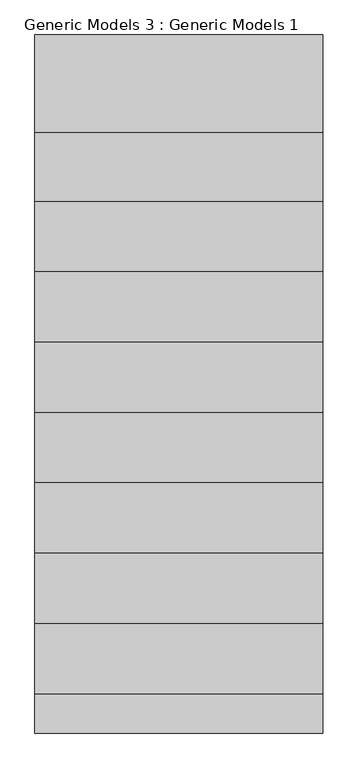
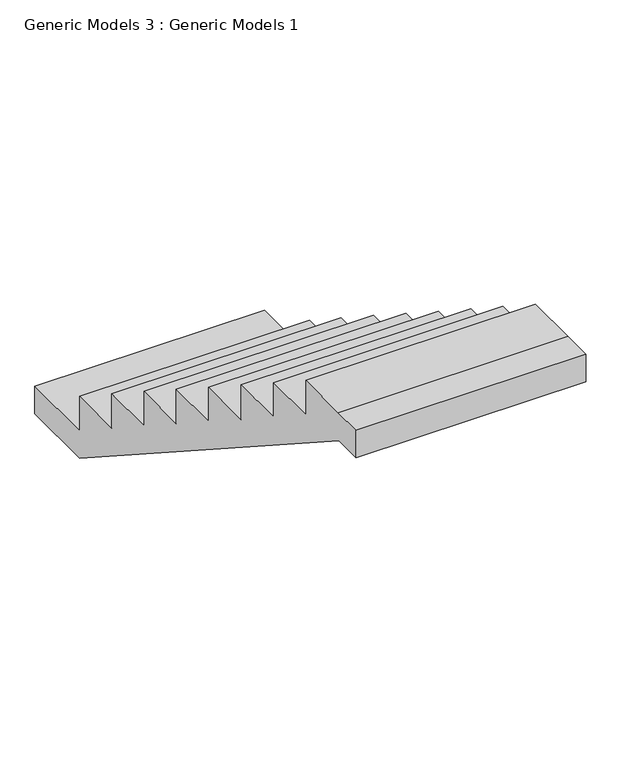
"""IFC4 building model written with IfcOpenShell, lengths in millimetres: proxy geometry, Generic Models 3 : Generic Models 1."""

from ifc_helpers import new_model, si_unit, frame, origin, place, context, project, spatial, polyline, outline, extrude, source, transform, mapped, element, save


def generic_models_3_generic_models_1_35d45e08(model_context):
    return source(origin(), model_context, "Body", "SweptSolid", [
        extrude(outline(polyline([(25295.484552, 175.0), (25295.484552, 0.0), (25670.484552, 0.0), (25670.484552, -140.0), (25295.484552, -140.0), (23135.484552, 1260.0), (22990.484552, 1260.0), (22990.484552, 1400.0), (23140.484552, 1400.0), (23410.484552, 1400.0), (23410.484552, 1225.0), (23680.484552, 1225.0), (23680.484552, 1050.0), (23950.484552, 1050.0), (23950.484552, 873.0), (24220.484552, 873.0), (24220.484552, 700.0), (24490.484552, 700.0), (24490.484552, 525.0), (24760.484552, 525.0), (24760.484552, 350.0), (25030.484552, 350.0), (25030.484552, 175.0), (25295.484552, 175.0)])), frame((82605.5816601, 0.0, 0.0), z_axis=(1.0, 0.0, 0.0), x_axis=(0.0, 1.0, 0.0)), (0.0, 0.0, 1.0), 1105.7161874),
    ])


if __name__ == "__main__":
    model = new_model("IFC4")
    model_context = context("Model", 3, world=origin())
    ifc_project = project(units=[si_unit("LENGTHUNIT", "METRE", prefix="MILLI")], contexts=[model_context])
    site = spatial("IfcSite", under=ifc_project)
    building = spatial("IfcBuilding", under=site)
    placement = place(None, origin())
    generic_models_3_generic_models_1_shape = generic_models_3_generic_models_1_35d45e08(model_context)
    element("IfcBuildingElementProxy", 1, Name="Generic Models 3 : Generic Models 1", ObjectType="Generic Models 3 : Generic Models 1", at=placement, inside=building, context=model_context, shape_type="MappedRepresentation", body=[
        mapped(generic_models_3_generic_models_1_shape, transform((0.0, 0.0, 0.0), x_axis=(1.0, 0.0, 0.0), y_axis=(0.0, 1.0, 0.0), z_axis=(0.0, 0.0, 1.0))),
    ])
    save(model, "model.ifc")

# Revit data of these elements
# Type "Generic Models 3 : Generic Models 1"
#   Type Mark = "Prefab_staircase"
